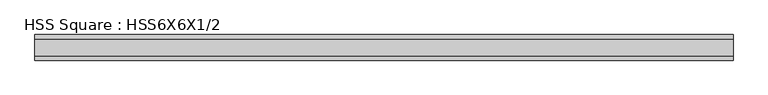
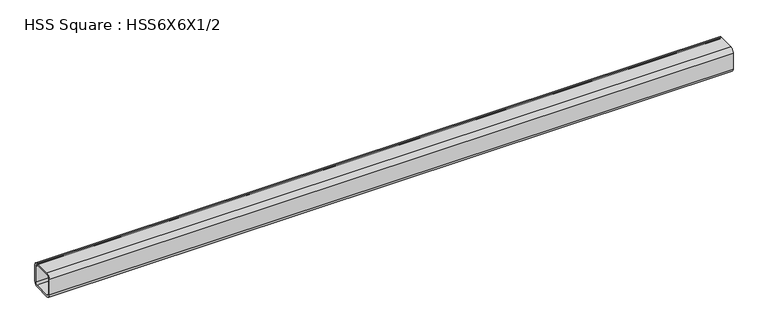
"""IFC4 building model written with IfcOpenShell, lengths in millimetres: member geometry, HSS Square : HSS6X6X1/2."""

import ifcopenshell
import ifcopenshell.guid

model = None  # the IFC model being written
_history = None  # IfcOwnerHistory: only IFC2X3 demands one
_inside = {}  # id of a spatial element -> (the spatial element, [elements in it])
_under = {}  # id of a project, library or spatial element -> (it, [spatial elements below it])
_declared = {}  # id of a project -> (the project, [libraries it declares])
_typed = {}  # id of a type object -> (the type object, [elements of that type])
_made_of = {}  # id of a material, layer set ... -> (it, [elements and type objects made of it])


def new_model(schema):
    """Start an empty IFC model of exactly this schema.

    Asked for "IFC4X3", IfcOpenShell would pick the latest addendum, in which some entities
    have other attributes; the version numbers below select the first issue.
    IFC2X3 requires an IfcOwnerHistory on every rooted entity: one is made here for all.
    """
    global model, _history
    if schema == "IFC4X3":
        model = ifcopenshell.file(schema_version=(4, 3, 0, 0))
    else:
        model = ifcopenshell.file(schema=schema)
    _inside.clear()
    _under.clear()
    _declared.clear()
    _typed.clear()
    _made_of.clear()
    _history = None
    if model.schema == "IFC2X3":
        org = make("IfcOrganization", Name="unknown")
        user = make(
            "IfcPersonAndOrganization",
            ThePerson=make("IfcPerson", FamilyName="unknown"),
            TheOrganization=org,
        )
        app = make(
            "IfcApplication",
            ApplicationDeveloper=org,
            Version="unknown",
            ApplicationFullName="unknown",
            ApplicationIdentifier="unknown",
        )
        _history = make(
            "IfcOwnerHistory",
            OwningUser=user,
            OwningApplication=app,
            ChangeAction="ADDED",
            CreationDate=0,
        )
    return model


def make(cls, **values):
    """One entity of the class cls with the attributes given. An attribute that is None is left unset."""
    return model.create_entity(
        cls, **{name: value for name, value in values.items() if value is not None}
    )


def rooted(cls, **values):
    """An entity with a GlobalId (a new one), such as an element, a storey or a relation."""
    return make(cls, GlobalId=ifcopenshell.guid.new(), OwnerHistory=_history, **values)


def si_unit(unit_type, name, prefix=None):
    """IfcSIUnit, for example si_unit("LENGTHUNIT", "METRE", prefix="MILLI")."""
    return make("IfcSIUnit", UnitType=unit_type, Prefix=prefix, Name=name)


def assignment(units):
    """IfcUnitAssignment: the units of a project."""
    return None if units is None else make("IfcUnitAssignment", Units=units)


def point(xyz):
    """IfcCartesianPoint."""
    return None if xyz is None else make("IfcCartesianPoint", Coordinates=xyz)


def direction(xyz):
    """IfcDirection."""
    return None if xyz is None else make("IfcDirection", DirectionRatios=xyz)


def frame(location, z_axis=None, x_axis=None):
    """IfcAxis2Placement3D, a coordinate frame: its origin and axes. An axis left out is left unset."""
    return make(
        "IfcAxis2Placement3D",
        Location=point(location),
        Axis=direction(z_axis),
        RefDirection=direction(x_axis),
    )


def frame_2d(location, x_axis=None):
    """IfcAxis2Placement2D, a coordinate frame in the plane: its origin and x axis."""
    return make(
        "IfcAxis2Placement2D", Location=point(location), RefDirection=direction(x_axis)
    )


def origin():
    """The frame at (0, 0, 0) with its axes left unset."""
    return frame((0.0, 0.0, 0.0))


def place(relative_to, where):
    """IfcLocalPlacement: puts the frame where relative to a parent placement (None: the world)."""
    return make(
        "IfcLocalPlacement", PlacementRelTo=relative_to, RelativePlacement=where
    )


def context(
    kind, dimensions, precision=None, world=None, true_north=None, identifier=None
):
    """IfcGeometricRepresentationContext, for example the 3D "Model" context."""
    return make(
        "IfcGeometricRepresentationContext",
        ContextIdentifier=identifier,
        ContextType=kind,
        CoordinateSpaceDimension=dimensions,
        Precision=precision,
        WorldCoordinateSystem=world,
        TrueNorth=true_north,
    )


def project(units=None, contexts=None):
    """IfcProject with its units and contexts."""
    return rooted(
        "IfcProject",
        Name="project",
        RepresentationContexts=contexts,
        UnitsInContext=assignment(units),
    )


def spatial(cls, under=None, at=None, **own):
    """A site, building, storey or space (cls), placed at a placement, below another one or the project."""
    s = rooted(cls, ObjectPlacement=at, **own)
    if under is not None:
        _under.setdefault(under.id(), (under, []))[1].append(s)
    return s


def polyline(points):
    """IfcPolyline through the points."""
    return make("IfcPolyline", Points=[point(p) for p in points])


def circle_curve(where, radius):
    """IfcCircle in the frame where."""
    return make("IfcCircle", Position=where, Radius=radius)


def trimmed(basis, trim1, trim2, sense, master):
    """IfcTrimmedCurve: the piece of a basis curve between two trims."""
    return make(
        "IfcTrimmedCurve",
        BasisCurve=basis,
        Trim1=trim1,
        Trim2=trim2,
        SenseAgreement=sense,
        MasterRepresentation=master,
    )


def segment(curve, same_sense, transition):
    """IfcCompositeCurveSegment."""
    return make(
        "IfcCompositeCurveSegment",
        Transition=transition,
        SameSense=same_sense,
        ParentCurve=curve,
    )


def composite_curve(segments, self_intersect=None):
    """IfcCompositeCurve: segments joined end to end."""
    return make("IfcCompositeCurve", Segments=segments, SelfIntersect=self_intersect)


def outline(outer, holes=None, kind="AREA"):
    """IfcArbitraryClosedProfileDef: a profile drawn as a closed curve; with holes, ...WithVoids."""
    if holes is None:
        return make("IfcArbitraryClosedProfileDef", ProfileType=kind, OuterCurve=outer)
    return make(
        "IfcArbitraryProfileDefWithVoids",
        ProfileType=kind,
        OuterCurve=outer,
        InnerCurves=holes,
    )


def extrude(swept, where, along, depth):
    """IfcExtrudedAreaSolid: the profile swept, set in the frame where, extruded along a direction by depth."""
    return make(
        "IfcExtrudedAreaSolid",
        SweptArea=swept,
        Position=where,
        ExtrudedDirection=direction(along),
        Depth=depth,
    )


def shape(context_of_items, identifier, shape_type, items):
    """IfcShapeRepresentation: the items that make up one representation, for example the "Body"."""
    return make(
        "IfcShapeRepresentation",
        ContextOfItems=context_of_items,
        RepresentationIdentifier=identifier,
        RepresentationType=shape_type,
        Items=items,
    )


def source(mapping_origin, context_of_items, identifier, shape_type, items):
    """IfcRepresentationMap: a shape defined once, which mapped items show again and again."""
    return make(
        "IfcRepresentationMap",
        MappingOrigin=mapping_origin,
        MappedRepresentation=shape(context_of_items, identifier, shape_type, items),
    )


def transform(
    local_origin,
    x_axis=None,
    y_axis=None,
    z_axis=None,
    scale=None,
    scale2=None,
    scale3=None,
    uniform=True,
):
    """IfcCartesianTransformationOperator3D, or its non-uniform kind. x_axis, y_axis, z_axis: its Axis1, 2, 3."""
    if uniform:
        return make(
            "IfcCartesianTransformationOperator3D",
            Axis1=direction(x_axis),
            Axis2=direction(y_axis),
            LocalOrigin=point(local_origin),
            Scale=scale,
            Axis3=direction(z_axis),
        )
    return make(
        "IfcCartesianTransformationOperator3DnonUniform",
        Axis1=direction(x_axis),
        Axis2=direction(y_axis),
        LocalOrigin=point(local_origin),
        Scale=scale,
        Axis3=direction(z_axis),
        Scale2=scale2,
        Scale3=scale3,
    )


def mapped(mapping_source, mapping_target):
    """IfcMappedItem: shows the shape of a source again, moved by a transform."""
    return make(
        "IfcMappedItem", MappingSource=mapping_source, MappingTarget=mapping_target
    )


def made_of(thing, what):
    """Note that an element or type object is made of a material, layer set ...; save() writes the relation."""
    if what is not None:
        _made_of.setdefault(what.id(), (what, []))[1].append(thing)
    return thing


def element(
    cls,
    number,
    at=None,
    inside=None,
    cuts=None,
    type_object=None,
    material=None,
    context=None,
    identifier="Body",
    shape_type=None,
    held_by="IfcProductDefinitionShape",
    body=None,
    shapes=None,
    **own,
):
    """One element of the class cls, such as IfcWall. Its Tag is "e" and its number.

    at: its placement. inside: the storey or other place that contains it. cuts: it is an
    opening in that element (IfcRelVoidsElement). A single representation is given by context,
    identifier, shape_type and body (its items); several are given by shapes. held_by: the class
    of the entity that holds the representations. save() writes the other relations.
    """
    e = rooted(cls, Tag="e%d" % number, ObjectPlacement=at, **own)
    if body is not None:
        shapes = [shape(context, identifier, shape_type, body)]
    if shapes is not None:
        e.Representation = make(held_by, Representations=shapes)
    if inside is not None:
        _inside.setdefault(inside.id(), (inside, []))[1].append(e)
    if cuts is not None:
        rooted(
            "IfcRelVoidsElement", RelatingBuildingElement=cuts, RelatedOpeningElement=e
        )
    if type_object is not None:
        _typed.setdefault(type_object.id(), (type_object, []))[1].append(e)
    return made_of(e, material)


def aggregate(whole, parts):
    """IfcRelAggregates: a whole, such as a stair, and the parts it consists of."""
    return rooted("IfcRelAggregates", RelatingObject=whole, RelatedObjects=parts)


def save(model, path):
    """Write the relations noted so far, then the file.

    IfcRelAggregates (storeys below a building ...), IfcRelContainedInSpatialStructure (elements
    in a storey), IfcRelDefinesByType, IfcRelAssociatesMaterial and IfcRelDeclares: one each for
    every whole, place, type object, material and project.
    """
    for whole, parts in _under.values():
        aggregate(whole, parts)
    for where, things in _inside.values():
        rooted(
            "IfcRelContainedInSpatialStructure",
            RelatedElements=things,
            RelatingStructure=where,
        )
    for kind, things in _typed.values():
        rooted("IfcRelDefinesByType", RelatedObjects=things, RelatingType=kind)
    for what, things in _made_of.values():
        rooted("IfcRelAssociatesMaterial", RelatedObjects=things, RelatingMaterial=what)
    for by, libraries in _declared.values():
        rooted("IfcRelDeclares", RelatingContext=by, RelatedDefinitions=libraries)
    model.write(path)


def hss_square_hss6x6x1_2_8f7afb5b(model_context):
    return source(origin(), model_context, "Body", "SweptSolid", [
        extrude(outline(composite_curve([segment(polyline([(76.2, 50.8), (76.2, -50.8)]), True, "CONTINUOUS"), segment(trimmed(circle_curve(frame_2d((50.8, -50.8)), 25.4), [point((76.2, -50.8))], [point((50.8, -76.2))], False, "CARTESIAN"), True, "CONTINUOUS"), segment(polyline([(50.8, -76.2), (-50.8, -76.2)]), True, "CONTINUOUS"), segment(trimmed(circle_curve(frame_2d((-50.8, -50.8)), 25.4), [point((-50.8, -76.2))], [point((-76.2, -50.8))], False, "CARTESIAN"), True, "CONTINUOUS"), segment(polyline([(-76.2, -50.8), (-76.2, 50.8)]), True, "CONTINUOUS"), segment(trimmed(circle_curve(frame_2d((-50.8, 50.8)), 25.4), [point((-76.2, 50.8))], [point((-50.8, 76.2))], False, "CARTESIAN"), True, "CONTINUOUS"), segment(polyline([(-50.8, 76.2), (50.8, 76.2)]), True, "CONTINUOUS"), segment(trimmed(circle_curve(frame_2d((50.8, 50.8)), 25.4), [point((50.8, 76.2))], [point((76.2, 50.8))], False, "CARTESIAN"), True, "CONTINUOUS")], self_intersect=False), holes=[composite_curve([segment(trimmed(circle_curve(frame_2d((-50.8, 50.8)), 12.7), [point((-50.8, 63.5))], [point((-63.5, 50.8))], True, "CARTESIAN"), True, "CONTINUOUS"), segment(polyline([(-63.5, 50.8), (-63.5, -50.8)]), True, "CONTINUOUS"), segment(trimmed(circle_curve(frame_2d((-50.8, -50.8)), 12.7), [point((-63.5, -50.8))], [point((-50.8, -63.5))], True, "CARTESIAN"), True, "CONTINUOUS"), segment(polyline([(-50.8, -63.5), (50.8, -63.5)]), True, "CONTINUOUS"), segment(trimmed(circle_curve(frame_2d((50.8, -50.8)), 12.7), [point((50.8, -63.5))], [point((63.5, -50.8))], True, "CARTESIAN"), True, "CONTINUOUS"), segment(polyline([(63.5, -50.8), (63.5, 50.8)]), True, "CONTINUOUS"), segment(trimmed(circle_curve(frame_2d((50.8, 50.8)), 12.7), [point((63.5, 50.8))], [point((50.8, 63.5))], True, "CARTESIAN"), True, "CONTINUOUS"), segment(polyline([(50.8, 63.5), (-50.8, 63.5)]), True, "CONTINUOUS")], self_intersect=False)]), frame((-2077.1683244, 0.0, 0.0), z_axis=(1.0, 0.0, 0.0), x_axis=(0.0, 1.0, 0.0)), (0.0, 0.0, 1.0), 4154.3366487),
    ])


if __name__ == "__main__":
    model = new_model("IFC4")
    model_context = context("Model", 3, world=origin())
    ifc_project = project(units=[si_unit("LENGTHUNIT", "METRE", prefix="MILLI")], contexts=[model_context])
    site = spatial("IfcSite", under=ifc_project)
    building = spatial("IfcBuilding", under=site)
    placement = place(None, origin())
    hss_square_hss6x6x1_2_shape = hss_square_hss6x6x1_2_8f7afb5b(model_context)
    element("IfcMember", 1, ObjectType="HSS Square : HSS6X6X1/2", at=placement, inside=building, context=model_context, shape_type="MappedRepresentation", body=[
        mapped(hss_square_hss6x6x1_2_shape, transform((0.0, 0.0, 0.0), x_axis=(1.0, 0.0, 0.0), y_axis=(0.0, 1.0, 0.0), z_axis=(0.0, 0.0, 1.0))),
    ])
    save(model, "model.ifc")

# Revit data of these elements
# Type "HSS Square : HSS6X6X1/2"
#   Section Name Key = "HSS 6X6X1/2"
#   Assembly Code = "B10"
#   Width = 6.000"
#   Wall Nominal Thickness = 0.500"
#   Wall Design Thickness = 0.465"
#   Torsional Moment of Inertia = 81.10 in⁴
#   Torsional Modulus = 28.10 in³
#   Section Area = 9.74 in²
#   Plastic Modulus weak axis = 19.80 in³
#   Plastic Modulus strong axis = 19.80 in³
#   Outer Fillet = 1.000"
#   Nominal Weight = 35.24 lbf/ft
#   Moment of Inertia weak axis = 48.30 in⁴
#   Moment of Inertia strong axis = 48.30 in⁴
#   Inner Fillet = 0.500"
#   Height = 6.000"
#   Elastic Modulus weak axis = 16.10 in³
#   Elastic Modulus strong axis = 16.10 in³
#   Centroid Vertical = 3.000"
#   Centroid Horizontal = 3.000"
#   Length [instance default] = 5' - 0"
#   Structural Material [instance default] = Steel ASTM A500, Grade B, Rectangular and Square
#   Principal Axes Angle = 0
# Element 1 (IfcMember, "HSS Square : HSS6X6X1/2")
#   Structural Material = Steel ASTM A36
#   Materials on its faces: "Steel ASTM A36"
# Materials
#   "Steel ASTM A500, Grade B, Rectangular and Square": class "Metal", colour RGB 199 199 199, transparency 0, Description = "Carbon steel", Cost = 0
#   "Steel ASTM A36": class "Metal", colour RGB 199 199 199, transparency 0, Description = "Structural steel, ASTM A36 Grade B, mill finish", Cost = 0
